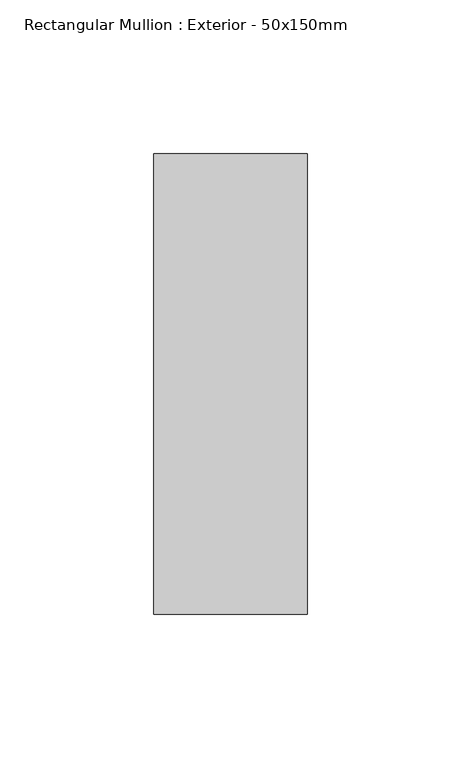
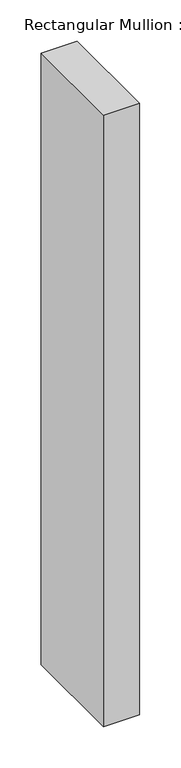
"""IFC4 building model written with IfcOpenShell, lengths in millimetres: member geometry, Rectangular Mullion : Exterior - 50x150mm."""

import ifcopenshell
import ifcopenshell.guid

model = None  # the IFC model being written
_history = None  # IfcOwnerHistory: only IFC2X3 demands one
_inside = {}  # id of a spatial element -> (the spatial element, [elements in it])
_under = {}  # id of a project, library or spatial element -> (it, [spatial elements below it])
_declared = {}  # id of a project -> (the project, [libraries it declares])
_typed = {}  # id of a type object -> (the type object, [elements of that type])
_made_of = {}  # id of a material, layer set ... -> (it, [elements and type objects made of it])


def new_model(schema):
    """Start an empty IFC model of exactly this schema.

    Asked for "IFC4X3", IfcOpenShell would pick the latest addendum, in which some entities
    have other attributes; the version numbers below select the first issue.
    IFC2X3 requires an IfcOwnerHistory on every rooted entity: one is made here for all.
    """
    global model, _history
    if schema == "IFC4X3":
        model = ifcopenshell.file(schema_version=(4, 3, 0, 0))
    else:
        model = ifcopenshell.file(schema=schema)
    _inside.clear()
    _under.clear()
    _declared.clear()
    _typed.clear()
    _made_of.clear()
    _history = None
    if model.schema == "IFC2X3":
        org = make("IfcOrganization", Name="unknown")
        user = make(
            "IfcPersonAndOrganization",
            ThePerson=make("IfcPerson", FamilyName="unknown"),
            TheOrganization=org,
        )
        app = make(
            "IfcApplication",
            ApplicationDeveloper=org,
            Version="unknown",
            ApplicationFullName="unknown",
            ApplicationIdentifier="unknown",
        )
        _history = make(
            "IfcOwnerHistory",
            OwningUser=user,
            OwningApplication=app,
            ChangeAction="ADDED",
            CreationDate=0,
        )
    return model


def make(cls, **values):
    """One entity of the class cls with the attributes given. An attribute that is None is left unset."""
    return model.create_entity(
        cls, **{name: value for name, value in values.items() if value is not None}
    )


def rooted(cls, **values):
    """An entity with a GlobalId (a new one), such as an element, a storey or a relation."""
    return make(cls, GlobalId=ifcopenshell.guid.new(), OwnerHistory=_history, **values)


def si_unit(unit_type, name, prefix=None):
    """IfcSIUnit, for example si_unit("LENGTHUNIT", "METRE", prefix="MILLI")."""
    return make("IfcSIUnit", UnitType=unit_type, Prefix=prefix, Name=name)


def assignment(units):
    """IfcUnitAssignment: the units of a project."""
    return None if units is None else make("IfcUnitAssignment", Units=units)


def point(xyz):
    """IfcCartesianPoint."""
    return None if xyz is None else make("IfcCartesianPoint", Coordinates=xyz)


def direction(xyz):
    """IfcDirection."""
    return None if xyz is None else make("IfcDirection", DirectionRatios=xyz)


def frame(location, z_axis=None, x_axis=None):
    """IfcAxis2Placement3D, a coordinate frame: its origin and axes. An axis left out is left unset."""
    return make(
        "IfcAxis2Placement3D",
        Location=point(location),
        Axis=direction(z_axis),
        RefDirection=direction(x_axis),
    )


def origin():
    """The frame at (0, 0, 0) with its axes left unset."""
    return frame((0.0, 0.0, 0.0))


def place(relative_to, where):
    """IfcLocalPlacement: puts the frame where relative to a parent placement (None: the world)."""
    return make(
        "IfcLocalPlacement", PlacementRelTo=relative_to, RelativePlacement=where
    )


def context(
    kind, dimensions, precision=None, world=None, true_north=None, identifier=None
):
    """IfcGeometricRepresentationContext, for example the 3D "Model" context."""
    return make(
        "IfcGeometricRepresentationContext",
        ContextIdentifier=identifier,
        ContextType=kind,
        CoordinateSpaceDimension=dimensions,
        Precision=precision,
        WorldCoordinateSystem=world,
        TrueNorth=true_north,
    )


def project(units=None, contexts=None):
    """IfcProject with its units and contexts."""
    return rooted(
        "IfcProject",
        Name="project",
        RepresentationContexts=contexts,
        UnitsInContext=assignment(units),
    )


def spatial(cls, under=None, at=None, **own):
    """A site, building, storey or space (cls), placed at a placement, below another one or the project."""
    s = rooted(cls, ObjectPlacement=at, **own)
    if under is not None:
        _under.setdefault(under.id(), (under, []))[1].append(s)
    return s


def polyline(points):
    """IfcPolyline through the points."""
    return make("IfcPolyline", Points=[point(p) for p in points])


def outline(outer, holes=None, kind="AREA"):
    """IfcArbitraryClosedProfileDef: a profile drawn as a closed curve; with holes, ...WithVoids."""
    if holes is None:
        return make("IfcArbitraryClosedProfileDef", ProfileType=kind, OuterCurve=outer)
    return make(
        "IfcArbitraryProfileDefWithVoids",
        ProfileType=kind,
        OuterCurve=outer,
        InnerCurves=holes,
    )


def extrude(swept, where, along, depth):
    """IfcExtrudedAreaSolid: the profile swept, set in the frame where, extruded along a direction by depth."""
    return make(
        "IfcExtrudedAreaSolid",
        SweptArea=swept,
        Position=where,
        ExtrudedDirection=direction(along),
        Depth=depth,
    )


def shape(context_of_items, identifier, shape_type, items):
    """IfcShapeRepresentation: the items that make up one representation, for example the "Body"."""
    return make(
        "IfcShapeRepresentation",
        ContextOfItems=context_of_items,
        RepresentationIdentifier=identifier,
        RepresentationType=shape_type,
        Items=items,
    )


def source(mapping_origin, context_of_items, identifier, shape_type, items):
    """IfcRepresentationMap: a shape defined once, which mapped items show again and again."""
    return make(
        "IfcRepresentationMap",
        MappingOrigin=mapping_origin,
        MappedRepresentation=shape(context_of_items, identifier, shape_type, items),
    )


def transform(
    local_origin,
    x_axis=None,
    y_axis=None,
    z_axis=None,
    scale=None,
    scale2=None,
    scale3=None,
    uniform=True,
):
    """IfcCartesianTransformationOperator3D, or its non-uniform kind. x_axis, y_axis, z_axis: its Axis1, 2, 3."""
    if uniform:
        return make(
            "IfcCartesianTransformationOperator3D",
            Axis1=direction(x_axis),
            Axis2=direction(y_axis),
            LocalOrigin=point(local_origin),
            Scale=scale,
            Axis3=direction(z_axis),
        )
    return make(
        "IfcCartesianTransformationOperator3DnonUniform",
        Axis1=direction(x_axis),
        Axis2=direction(y_axis),
        LocalOrigin=point(local_origin),
        Scale=scale,
        Axis3=direction(z_axis),
        Scale2=scale2,
        Scale3=scale3,
    )


def mapped(mapping_source, mapping_target):
    """IfcMappedItem: shows the shape of a source again, moved by a transform."""
    return make(
        "IfcMappedItem", MappingSource=mapping_source, MappingTarget=mapping_target
    )


def made_of(thing, what):
    """Note that an element or type object is made of a material, layer set ...; save() writes the relation."""
    if what is not None:
        _made_of.setdefault(what.id(), (what, []))[1].append(thing)
    return thing


def element(
    cls,
    number,
    at=None,
    inside=None,
    cuts=None,
    type_object=None,
    material=None,
    context=None,
    identifier="Body",
    shape_type=None,
    held_by="IfcProductDefinitionShape",
    body=None,
    shapes=None,
    **own,
):
    """One element of the class cls, such as IfcWall. Its Tag is "e" and its number.

    at: its placement. inside: the storey or other place that contains it. cuts: it is an
    opening in that element (IfcRelVoidsElement). A single representation is given by context,
    identifier, shape_type and body (its items); several are given by shapes. held_by: the class
    of the entity that holds the representations. save() writes the other relations.
    """
    e = rooted(cls, Tag="e%d" % number, ObjectPlacement=at, **own)
    if body is not None:
        shapes = [shape(context, identifier, shape_type, body)]
    if shapes is not None:
        e.Representation = make(held_by, Representations=shapes)
    if inside is not None:
        _inside.setdefault(inside.id(), (inside, []))[1].append(e)
    if cuts is not None:
        rooted(
            "IfcRelVoidsElement", RelatingBuildingElement=cuts, RelatedOpeningElement=e
        )
    if type_object is not None:
        _typed.setdefault(type_object.id(), (type_object, []))[1].append(e)
    return made_of(e, material)


def aggregate(whole, parts):
    """IfcRelAggregates: a whole, such as a stair, and the parts it consists of."""
    return rooted("IfcRelAggregates", RelatingObject=whole, RelatedObjects=parts)


def save(model, path):
    """Write the relations noted so far, then the file.

    IfcRelAggregates (storeys below a building ...), IfcRelContainedInSpatialStructure (elements
    in a storey), IfcRelDefinesByType, IfcRelAssociatesMaterial and IfcRelDeclares: one each for
    every whole, place, type object, material and project.
    """
    for whole, parts in _under.values():
        aggregate(whole, parts)
    for where, things in _inside.values():
        rooted(
            "IfcRelContainedInSpatialStructure",
            RelatedElements=things,
            RelatingStructure=where,
        )
    for kind, things in _typed.values():
        rooted("IfcRelDefinesByType", RelatedObjects=things, RelatingType=kind)
    for what, things in _made_of.values():
        rooted("IfcRelAssociatesMaterial", RelatedObjects=things, RelatingMaterial=what)
    for by, libraries in _declared.values():
        rooted("IfcRelDeclares", RelatingContext=by, RelatedDefinitions=libraries)
    model.write(path)


def rectangular_mullion_exterior_50x150mm_5b23c5d7(model_context):
    return source(origin(), model_context, "Body", "SweptSolid", [
        extrude(outline(polyline([(0.0, 0.0), (0.0, -150.0), (-50.0, -150.0), (-50.0, 0.0), (0.0, 0.0)])), frame((0.0, 0.0, -900.0), z_axis=(0.0, 0.0, 1.0), x_axis=(1.0, 0.0, 0.0)), (0.0, 0.0, 1.0), 900.0),
    ])


if __name__ == "__main__":
    model = new_model("IFC4")
    model_context = context("Model", 3, world=origin())
    ifc_project = project(units=[si_unit("LENGTHUNIT", "METRE", prefix="MILLI")], contexts=[model_context])
    site = spatial("IfcSite", under=ifc_project)
    building = spatial("IfcBuilding", under=site)
    placement = place(None, origin())
    rectangular_mullion_exterior_50x150mm_shape = rectangular_mullion_exterior_50x150mm_5b23c5d7(model_context)
    element("IfcMember", 1, ObjectType="Rectangular Mullion : Exterior - 50x150mm", at=placement, inside=building, context=model_context, shape_type="MappedRepresentation", body=[
        mapped(rectangular_mullion_exterior_50x150mm_shape, transform((0.0, 0.0, 0.0), x_axis=(1.0, 0.0, 0.0), y_axis=(0.0, 1.0, 0.0), z_axis=(0.0, 0.0, 1.0))),
    ])
    save(model, "model.ifc")

# Revit data of these elements
# Project information
#   Template Version = "DanEDU Building template ver. 2018.0420.0"
#   Client Name = "Test Project"
#   Project Address = "Enter address here"
#   Project Name = "3 Stories"
#   Project Number = "Number"
#   Current Version = "0.0.0"
#   SR Document GUID = "3eb9317e-835d-4f79-8926-4d15b96bc824"
# Type "Rectangular Mullion : Exterior - 50x150mm"
#   built-in parameter 1007351 = -0.246063 (stored number, unit not read)
#   built-in parameter 1007304 = 0.492126 (stored number, unit not read)
#   built-in parameter 1007301 = 0.082021 (stored number, unit not read)
#   built-in parameter 1007300 = 0.082021 (stored number, unit not read)
# Element 1 (IfcMember, "Rectangular Mullion : Exterior - 50x150mm")
#   Materials on its faces: "Default Frame/Mullion (Interior/Exterior)"
# Materials
#   "Default Frame/Mullion (Interior/Exterior)": class "Generic", colour RGB 205 205 205, transparency 0, Description = "Udefineret karm/ramme materiale", Cost = 0
